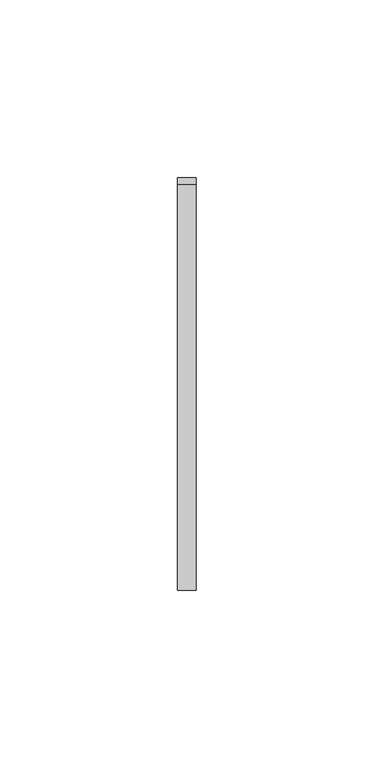
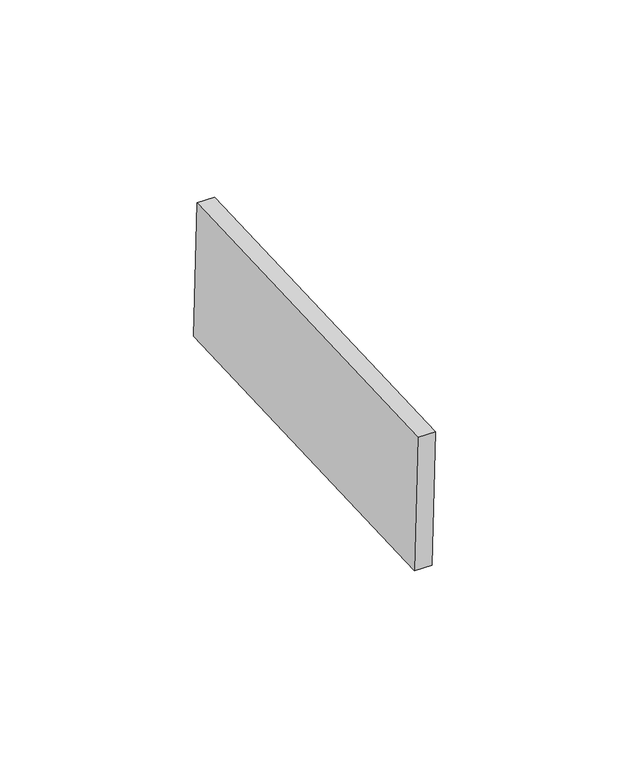
"""IFC4 building model written with IfcOpenShell, lengths in millimetres: proxy geometry, Inner panel:Inner panel:1:Inner panel:1 : Inner panel:Inner panel:300324:2:Inner panel:1:Inner panel:1 : Inner panel:Inner panel:300324:2 : Inner panel:Inner panel:1:Inner panel:1 : Inner panel:Inner panel:300324:300043:51 : Inner panel:Inner panel:1:Inner panel:1 : Inner panel:Inner panel:300324:2:Inner panel:1:Inner panel:1 : Inner panel:Inner panel:300324:2 : Inner panel:Inner panel:1:Inner panel:1 : Inner panel:Inner panel:300324:300043:308120."""

import ifcopenshell
import ifcopenshell.guid

model = None  # the IFC model being written
_history = None  # IfcOwnerHistory: only IFC2X3 demands one
_inside = {}  # id of a spatial element -> (the spatial element, [elements in it])
_under = {}  # id of a project, library or spatial element -> (it, [spatial elements below it])
_declared = {}  # id of a project -> (the project, [libraries it declares])
_typed = {}  # id of a type object -> (the type object, [elements of that type])
_made_of = {}  # id of a material, layer set ... -> (it, [elements and type objects made of it])


def new_model(schema):
    """Start an empty IFC model of exactly this schema.

    Asked for "IFC4X3", IfcOpenShell would pick the latest addendum, in which some entities
    have other attributes; the version numbers below select the first issue.
    IFC2X3 requires an IfcOwnerHistory on every rooted entity: one is made here for all.
    """
    global model, _history
    if schema == "IFC4X3":
        model = ifcopenshell.file(schema_version=(4, 3, 0, 0))
    else:
        model = ifcopenshell.file(schema=schema)
    _inside.clear()
    _under.clear()
    _declared.clear()
    _typed.clear()
    _made_of.clear()
    _history = None
    if model.schema == "IFC2X3":
        org = make("IfcOrganization", Name="unknown")
        user = make(
            "IfcPersonAndOrganization",
            ThePerson=make("IfcPerson", FamilyName="unknown"),
            TheOrganization=org,
        )
        app = make(
            "IfcApplication",
            ApplicationDeveloper=org,
            Version="unknown",
            ApplicationFullName="unknown",
            ApplicationIdentifier="unknown",
        )
        _history = make(
            "IfcOwnerHistory",
            OwningUser=user,
            OwningApplication=app,
            ChangeAction="ADDED",
            CreationDate=0,
        )
    return model


def make(cls, **values):
    """One entity of the class cls with the attributes given. An attribute that is None is left unset."""
    return model.create_entity(
        cls, **{name: value for name, value in values.items() if value is not None}
    )


def rooted(cls, **values):
    """An entity with a GlobalId (a new one), such as an element, a storey or a relation."""
    return make(cls, GlobalId=ifcopenshell.guid.new(), OwnerHistory=_history, **values)


def si_unit(unit_type, name, prefix=None):
    """IfcSIUnit, for example si_unit("LENGTHUNIT", "METRE", prefix="MILLI")."""
    return make("IfcSIUnit", UnitType=unit_type, Prefix=prefix, Name=name)


def assignment(units):
    """IfcUnitAssignment: the units of a project."""
    return None if units is None else make("IfcUnitAssignment", Units=units)


def point(xyz):
    """IfcCartesianPoint."""
    return None if xyz is None else make("IfcCartesianPoint", Coordinates=xyz)


def direction(xyz):
    """IfcDirection."""
    return None if xyz is None else make("IfcDirection", DirectionRatios=xyz)


def frame(location, z_axis=None, x_axis=None):
    """IfcAxis2Placement3D, a coordinate frame: its origin and axes. An axis left out is left unset."""
    return make(
        "IfcAxis2Placement3D",
        Location=point(location),
        Axis=direction(z_axis),
        RefDirection=direction(x_axis),
    )


def origin():
    """The frame at (0, 0, 0) with its axes left unset."""
    return frame((0.0, 0.0, 0.0))


def place(relative_to, where):
    """IfcLocalPlacement: puts the frame where relative to a parent placement (None: the world)."""
    return make(
        "IfcLocalPlacement", PlacementRelTo=relative_to, RelativePlacement=where
    )


def context(
    kind, dimensions, precision=None, world=None, true_north=None, identifier=None
):
    """IfcGeometricRepresentationContext, for example the 3D "Model" context."""
    return make(
        "IfcGeometricRepresentationContext",
        ContextIdentifier=identifier,
        ContextType=kind,
        CoordinateSpaceDimension=dimensions,
        Precision=precision,
        WorldCoordinateSystem=world,
        TrueNorth=true_north,
    )


def project(units=None, contexts=None):
    """IfcProject with its units and contexts."""
    return rooted(
        "IfcProject",
        Name="project",
        RepresentationContexts=contexts,
        UnitsInContext=assignment(units),
    )


def spatial(cls, under=None, at=None, **own):
    """A site, building, storey or space (cls), placed at a placement, below another one or the project."""
    s = rooted(cls, ObjectPlacement=at, **own)
    if under is not None:
        _under.setdefault(under.id(), (under, []))[1].append(s)
    return s


def polyline(points):
    """IfcPolyline through the points."""
    return make("IfcPolyline", Points=[point(p) for p in points])


def outline(outer, holes=None, kind="AREA"):
    """IfcArbitraryClosedProfileDef: a profile drawn as a closed curve; with holes, ...WithVoids."""
    if holes is None:
        return make("IfcArbitraryClosedProfileDef", ProfileType=kind, OuterCurve=outer)
    return make(
        "IfcArbitraryProfileDefWithVoids",
        ProfileType=kind,
        OuterCurve=outer,
        InnerCurves=holes,
    )


def extrude(swept, where, along, depth):
    """IfcExtrudedAreaSolid: the profile swept, set in the frame where, extruded along a direction by depth."""
    return make(
        "IfcExtrudedAreaSolid",
        SweptArea=swept,
        Position=where,
        ExtrudedDirection=direction(along),
        Depth=depth,
    )


def shape(context_of_items, identifier, shape_type, items):
    """IfcShapeRepresentation: the items that make up one representation, for example the "Body"."""
    return make(
        "IfcShapeRepresentation",
        ContextOfItems=context_of_items,
        RepresentationIdentifier=identifier,
        RepresentationType=shape_type,
        Items=items,
    )


def source(mapping_origin, context_of_items, identifier, shape_type, items):
    """IfcRepresentationMap: a shape defined once, which mapped items show again and again."""
    return make(
        "IfcRepresentationMap",
        MappingOrigin=mapping_origin,
        MappedRepresentation=shape(context_of_items, identifier, shape_type, items),
    )


def transform(
    local_origin,
    x_axis=None,
    y_axis=None,
    z_axis=None,
    scale=None,
    scale2=None,
    scale3=None,
    uniform=True,
):
    """IfcCartesianTransformationOperator3D, or its non-uniform kind. x_axis, y_axis, z_axis: its Axis1, 2, 3."""
    if uniform:
        return make(
            "IfcCartesianTransformationOperator3D",
            Axis1=direction(x_axis),
            Axis2=direction(y_axis),
            LocalOrigin=point(local_origin),
            Scale=scale,
            Axis3=direction(z_axis),
        )
    return make(
        "IfcCartesianTransformationOperator3DnonUniform",
        Axis1=direction(x_axis),
        Axis2=direction(y_axis),
        LocalOrigin=point(local_origin),
        Scale=scale,
        Axis3=direction(z_axis),
        Scale2=scale2,
        Scale3=scale3,
    )


def mapped(mapping_source, mapping_target):
    """IfcMappedItem: shows the shape of a source again, moved by a transform."""
    return make(
        "IfcMappedItem", MappingSource=mapping_source, MappingTarget=mapping_target
    )


def made_of(thing, what):
    """Note that an element or type object is made of a material, layer set ...; save() writes the relation."""
    if what is not None:
        _made_of.setdefault(what.id(), (what, []))[1].append(thing)
    return thing


def element(
    cls,
    number,
    at=None,
    inside=None,
    cuts=None,
    type_object=None,
    material=None,
    context=None,
    identifier="Body",
    shape_type=None,
    held_by="IfcProductDefinitionShape",
    body=None,
    shapes=None,
    **own,
):
    """One element of the class cls, such as IfcWall. Its Tag is "e" and its number.

    at: its placement. inside: the storey or other place that contains it. cuts: it is an
    opening in that element (IfcRelVoidsElement). A single representation is given by context,
    identifier, shape_type and body (its items); several are given by shapes. held_by: the class
    of the entity that holds the representations. save() writes the other relations.
    """
    e = rooted(cls, Tag="e%d" % number, ObjectPlacement=at, **own)
    if body is not None:
        shapes = [shape(context, identifier, shape_type, body)]
    if shapes is not None:
        e.Representation = make(held_by, Representations=shapes)
    if inside is not None:
        _inside.setdefault(inside.id(), (inside, []))[1].append(e)
    if cuts is not None:
        rooted(
            "IfcRelVoidsElement", RelatingBuildingElement=cuts, RelatedOpeningElement=e
        )
    if type_object is not None:
        _typed.setdefault(type_object.id(), (type_object, []))[1].append(e)
    return made_of(e, material)


def aggregate(whole, parts):
    """IfcRelAggregates: a whole, such as a stair, and the parts it consists of."""
    return rooted("IfcRelAggregates", RelatingObject=whole, RelatedObjects=parts)


def save(model, path):
    """Write the relations noted so far, then the file.

    IfcRelAggregates (storeys below a building ...), IfcRelContainedInSpatialStructure (elements
    in a storey), IfcRelDefinesByType, IfcRelAssociatesMaterial and IfcRelDeclares: one each for
    every whole, place, type object, material and project.
    """
    for whole, parts in _under.values():
        aggregate(whole, parts)
    for where, things in _inside.values():
        rooted(
            "IfcRelContainedInSpatialStructure",
            RelatedElements=things,
            RelatingStructure=where,
        )
    for kind, things in _typed.values():
        rooted("IfcRelDefinesByType", RelatedObjects=things, RelatingType=kind)
    for what, things in _made_of.values():
        rooted("IfcRelAssociatesMaterial", RelatedObjects=things, RelatingMaterial=what)
    for by, libraries in _declared.values():
        rooted("IfcRelDeclares", RelatingContext=by, RelatedDefinitions=libraries)
    model.write(path)


def generic_models_8d6f5dad(model_context):
    return source(origin(), model_context, "Body", "SweptSolid", [
        extrude(outline(polyline([(0.0, -114.2999999), (0.0, 0.0), (5.2138089, 0.0), (5.2138089, -114.2999999), (0.0, -114.2999999)])), frame((593936.595117, -566950.1308393, 8857.6957503), z_axis=(0.0, -0.04163054471215927, 0.9991330730923529), x_axis=(-1.0, 0.0, 0.0)), (0.0, 0.0, 1.0), 43.2233908),
    ])


if __name__ == "__main__":
    model = new_model("IFC4")
    model_context = context("Model", 3, world=origin())
    ifc_project = project(units=[si_unit("LENGTHUNIT", "METRE", prefix="MILLI")], contexts=[model_context])
    site = spatial("IfcSite", under=ifc_project)
    building = spatial("IfcBuilding", under=site)
    placement = place(None, origin())
    generic_models_shape = generic_models_8d6f5dad(model_context)
    element("IfcBuildingElementProxy", 1, Name="Inner panel:Inner panel:1:Inner panel:1 : Inner panel:Inner panel:300324:2:Inner panel:1:Inner panel:1 : Inner panel:Inner panel:300324:2 : Inner panel:Inner panel:1:Inner panel:1 : Inner panel:Inner panel:300324:300043:51 : Inner panel:Inner panel:1:Inner panel:1 : Inner panel:Inner panel:300324:2:Inner panel:1:Inner panel:1 : Inner panel:Inner panel:300324:2 : Inner panel:Inner panel:1:Inner panel:1 : Inner panel:Inner panel:300324:300043:308120", ObjectType="Inner panel:Inner panel:1:Inner panel:1 : Inner panel:Inner panel:300324:2:Inner panel:1:Inner panel:1 : Inner panel:Inner panel:300324:2 : Inner panel:Inner panel:1:Inner panel:1 : Inner panel:Inner panel:300324:300043:51 : Inner panel:Inner panel:1:Inner panel:1 : Inner panel:Inner panel:300324:2:Inner panel:1:Inner panel:1 : Inner panel:Inner panel:300324:2 : Inner panel:Inner panel:1:Inner panel:1 : Inner panel:Inner panel:300324:300043:308120", at=placement, inside=building, context=model_context, shape_type="MappedRepresentation", body=[
        mapped(generic_models_shape, transform((0.0, 0.0, 0.0), x_axis=(1.0, 0.0, 0.0), y_axis=(0.0, 1.0, 0.0), z_axis=(0.0, 0.0, 1.0))),
    ])
    save(model, "model.ifc")

# Revit data of these elements
# Type "Inner panel:Inner panel:1:Inner panel:1 : Inner panel:Inner panel:300324:2:Inner panel:1:Inner panel:1 : Inner panel:Inner panel:300324:2 : Inner panel:Inner panel:1:Inner panel:1 : Inner panel:Inner panel:300324:300043:51 : Inner panel:Inner panel:1:Inner panel:1 : Inner panel:Inner panel:300324:2:Inner panel:1:Inner panel:1 : Inner panel:Inner panel:300324:2 : Inner panel:Inner panel:1:Inner panel:1 : Inner panel:Inner panel:300324:300043:308120"
#   NameOverride = "Inner panel:Inner panel:1:Inner panel:1 : Inner panel:Inner panel:300324:2:Inner panel:1:Inner panel:1 : Inner panel:Inner panel:300324:2 : Inner panel:Inner panel:1:Inner panel:1 : Inner panel:Inner panel:300324:300043:308120"
#   ObjectTypeOverride = "Inner panel:1:Inner panel:1 : Inner panel:Inner panel:300324:2 : Inner panel:Inner panel:1:Inner panel:1 : Inner panel:Inner panel:300324:300043"
#   Reference = "Inner panel"
#   Tag = "308120"
# Element 1 (IfcBuildingElementProxy, "Inner panel:Inner panel:1:Inner panel:1 : Inner panel:Inner panel:300324:2:Inner panel:1:Inner panel:1 : Inner panel:Inner panel:300324:2 : Inner panel:Inner panel:1:Inner panel:1 : Inner panel:Inner panel:300324:300043:51 : Inner panel:Inner panel:1:Inner panel:1 : Inner panel:Inner panel:300324:2:Inner panel:1:Inner panel:1 : Inner panel:Inner panel:300324:2 : Inner panel:Inner panel:1:Inner panel:1 : Inner panel:Inner panel:300324:300043:308120")
#   Materials on its faces: "SLIDING CLIP"
# Materials
#   "SLIDING CLIP": class "Generic", colour RGB 120 120 120, transparency 0, Cost = 0
